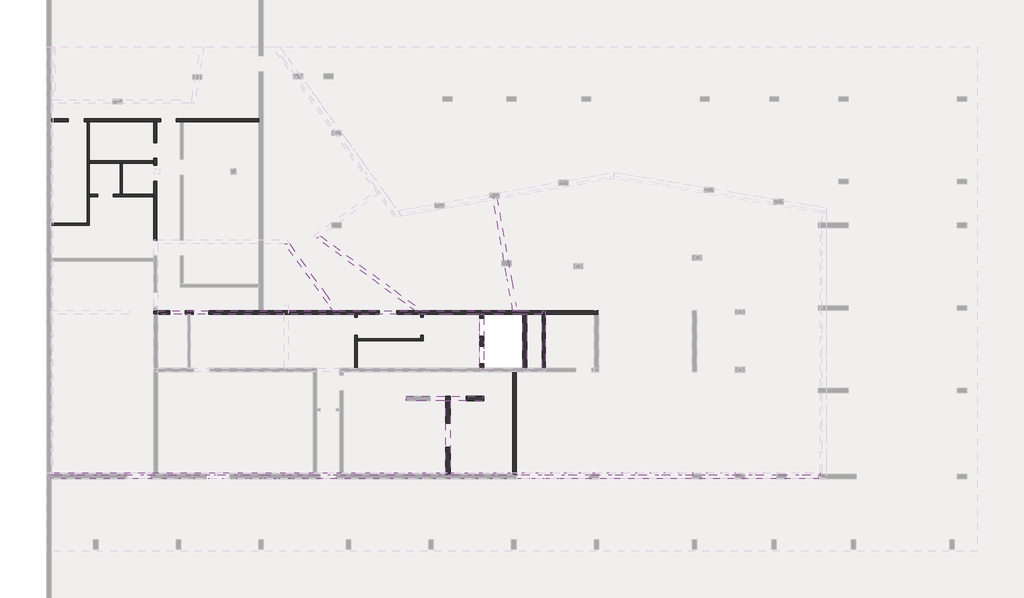
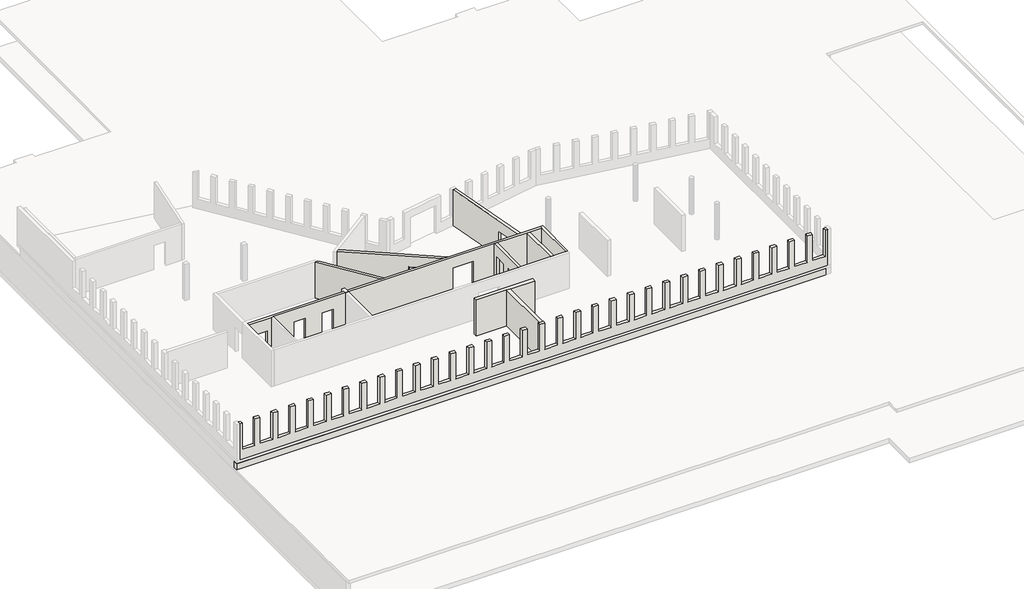
# One storey, part 2 of 4: 29 walls.
"""IFC4 building model written with IfcOpenShell, lengths in millimetres."""

from ifc_helpers import new_model, si_unit, frame, origin, place, context, project, spatial, polyline, outline, extrude, faceted_brep, element, save

model = new_model("IFC4")

# Units and contexts
model_context = context("Model", 3, world=origin())
ifc_project = project(units=[si_unit("LENGTHUNIT", "METRE", prefix="MILLI")], contexts=[model_context])

# Site, building, storey
site = spatial("IfcSite", under=ifc_project)
building = spatial("IfcBuilding", under=site)
storey = spatial("IfcBuildingStorey", under=building, Name="01_UG_OKFB_-4,20", Elevation=-4200.0)

# Walls
placement = place(None, origin())
element("IfcWall", 1, ObjectType="5dki Lochfassade 26cm C30/37", at=placement, inside=storey, context=model_context, shape_type="Brep", body=[
    faceted_brep([(49396.9999991, 130.0010483, 710.0), (49396.9999991, 130.0010483, 3060.0), (49603.9991101, 130.0010486, 3060.0), (49603.9991101, 130.0010486, -150.0), (25766.9999915, 130.0010117, -150.0), (25466.9999915, 130.0010113, -150.0), (130.0010047, 130.000972, -150.0), (130.0010047, 130.000972, 3060.0), (317.0000012, 130.0009723, 3060.0), (316.999997, 130.0009723, 710.0), (1397.0000012, 130.000974, 710.0), (1397.0000069, 130.000974, 3060.0), (1816.9999991, 130.0009747, 3060.0), (1817.0000028, 130.0009747, 710.0), (2896.9999991, 130.0009763, 710.0), (2897.0000017, 130.0009763, 3060.0), (3316.9999991, 130.000977, 3060.0), (3316.9999977, 130.000977, 710.0), (4396.9999991, 130.0009787, 710.0), (4396.9999966, 130.0009787, 3060.0), (4816.9999991, 130.0009793, 3060.0), (4816.9999991, 130.0009793, 710.0), (5896.9999991, 130.000981, 710.0), (5896.9999991, 130.000981, 3060.0), (6316.9999991, 130.0009816, 3060.0), (6316.9999991, 130.0009816, 710.0), (7396.9999991, 130.0009833, 710.0), (7396.9999991, 130.0009833, 3060.0), (7816.9999991, 130.0009839, 3060.0), (7816.9999991, 130.0009839, 710.0), (8896.9999991, 130.0009856, 710.0), (8896.9999991, 130.0009856, 3060.0), (9316.9999991, 130.0009863, 3060.0), (9316.9999991, 130.0009863, 710.0), (10396.9999991, 130.0009879, 710.0), (10396.9999991, 130.0009879, 3060.0), (10816.9999991, 130.0009886, 3060.0), (10816.9999991, 130.0009886, 710.0), (11896.9999991, 130.0009903, 710.0), (11896.9999991, 130.0009903, 3060.0), (12316.9999991, 130.0009909, 3060.0), (12316.9999991, 130.0009909, 710.0), (13396.9999991, 130.0009926, 710.0), (13396.9999991, 130.0009926, 3060.0), (13816.9999991, 130.0009932, 3060.0), (13816.9999991, 130.0009932, 710.0), (14896.9999991, 130.0009949, 710.0), (14896.9999991, 130.0009949, 3060.0), (15316.9999991, 130.0009956, 3060.0), (15316.9999991, 130.0009956, 710.0), (16396.9999991, 130.0009972, 710.0), (16396.9999991, 130.0009972, 3060.0), (16816.9999991, 130.0009979, 3060.0), (16816.9999991, 130.0009979, 710.0), (17896.9999991, 130.0009996, 710.0), (17896.9999991, 130.0009996, 3060.0), (18316.9999991, 130.0010002, 3060.0), (18316.9999991, 130.0010002, 710.0), (19396.9999991, 130.0010019, 710.0), (19396.9999991, 130.0010019, 3060.0), (19816.9999991, 130.0010025, 3060.0), (19816.9999991, 130.0010025, 710.0), (20896.9999991, 130.0010042, 710.0), (20896.9999991, 130.0010042, 3060.0), (21316.9999991, 130.0010048, 3060.0), (21316.9999991, 130.0010048, 710.0), (22396.9999991, 130.0010065, 710.0), (22396.9999991, 130.0010065, 3060.0), (22816.9999991, 130.0010072, 3060.0), (22816.9999991, 130.0010072, 710.0), (23896.9999991, 130.0010088, 710.0), (23896.9999991, 130.0010088, 3060.0), (24316.9999991, 130.0010095, 3060.0), (24316.9999991, 130.0010095, 710.0), (25396.9999991, 130.0010112, 710.0), (25396.9999991, 130.0010112, 3060.0), (25466.9999915, 130.0010113, 3060.0), (25766.9999915, 130.0010117, 3060.0), (25816.9999991, 130.0010118, 3060.0), (25816.9999991, 130.0010118, 710.0), (26896.9999991, 130.0010135, 710.0), (26896.9999991, 130.0010135, 3060.0), (27316.9999991, 130.0010141, 3060.0), (27316.9999991, 130.0010141, 710.0), (28396.9999991, 130.0010158, 710.0), (28396.9999991, 130.0010158, 3060.0), (28816.9999991, 130.0010165, 3060.0), (28816.9999991, 130.0010165, 710.0), (29896.9999991, 130.0010181, 710.0), (29896.9999991, 130.0010181, 3060.0), (30316.9999991, 130.0010188, 3060.0), (30316.9999991, 130.0010188, 710.0), (31396.9999991, 130.0010205, 710.0), (31396.9999991, 130.0010205, 3060.0), (31816.9999991, 130.0010211, 3060.0), (31816.9999991, 130.0010211, 710.0), (32896.9999991, 130.0010228, 710.0), (32896.9999991, 130.0010228, 3060.0), (33316.9999991, 130.0010234, 3060.0), (33316.9999991, 130.0010234, 710.0), (34396.9999991, 130.0010251, 710.0), (34396.9999991, 130.0010251, 3060.0), (34816.9999991, 130.0010258, 3060.0), (34816.9999991, 130.0010258, 710.0), (35896.9999991, 130.0010274, 710.0), (35896.9999991, 130.0010274, 3060.0), (36316.9999991, 130.0010281, 3060.0), (36316.9999991, 130.0010281, 710.0), (37396.9999991, 130.0010297, 710.0), (37396.9999991, 130.0010297, 3060.0), (37816.9999991, 130.0010304, 3060.0), (37816.9999991, 130.0010304, 710.0), (38896.9999991, 130.0010321, 710.0), (38896.9999991, 130.0010321, 3060.0), (39316.9999991, 130.0010327, 3060.0), (39316.9999991, 130.0010327, 710.0), (40396.9999991, 130.0010344, 710.0), (40396.9999991, 130.0010344, 3060.0), (40816.9999991, 130.001035, 3060.0), (40816.9999991, 130.001035, 710.0), (41896.9999991, 130.0010367, 710.0), (41896.9999991, 130.0010367, 3060.0), (42316.9999991, 130.0010374, 3060.0), (42316.9999991, 130.0010374, 710.0), (43396.9999991, 130.001039, 710.0), (43396.9999991, 130.001039, 3060.0), (43816.9999991, 130.0010397, 3060.0), (43816.9999991, 130.0010397, 710.0), (44896.9999991, 130.0010414, 710.0), (44896.9999991, 130.0010414, 3060.0), (45316.9999991, 130.001042, 3060.0), (45316.9999991, 130.001042, 710.0), (46396.9999991, 130.0010437, 710.0), (46396.9999991, 130.0010437, 3060.0), (46816.9999991, 130.0010443, 3060.0), (46816.9999991, 130.0010443, 710.0), (47896.9999991, 130.001046, 710.0), (47896.9999991, 130.001046, 3060.0), (48316.9999991, 130.0010467, 3060.0), (48316.9999991, 130.0010467, 710.0), (49603.9991105, -129.9989514, 3060.0), (49396.9999995, -129.9989517, 3060.0), (49396.9999995, -129.9989517, 710.0), (48316.9999995, -129.9989533, 710.0), (48316.9999995, -129.9989533, 3060.0), (47896.9999995, -129.998954, 3060.0), (47896.9999995, -129.998954, 710.0), (46816.9999995, -129.9989557, 710.0), (46816.9999995, -129.9989557, 3060.0), (46396.9999995, -129.9989563, 3060.0), (46396.9999995, -129.9989563, 710.0), (45316.9999995, -129.998958, 710.0), (45316.9999995, -129.998958, 3060.0), (44896.9999995, -129.9989586, 3060.0), (44896.9999995, -129.9989586, 710.0), (43816.9999995, -129.9989603, 710.0), (43816.9999995, -129.9989603, 3060.0), (43396.9999995, -129.998961, 3060.0), (43396.9999995, -129.998961, 710.0), (42316.9999995, -129.9989626, 710.0), (42316.9999995, -129.9989626, 3060.0), (41896.9999995, -129.9989633, 3060.0), (41896.9999995, -129.9989633, 710.0), (40816.9999995, -129.998965, 710.0), (40816.9999995, -129.998965, 3060.0), (40396.9999995, -129.9989656, 3060.0), (40396.9999995, -129.9989656, 710.0), (39316.9999995, -129.9989673, 710.0), (39316.9999995, -129.9989673, 3060.0), (38896.9999995, -129.9989679, 3060.0), (38896.9999995, -129.9989679, 710.0), (37816.9999995, -129.9989696, 710.0), (37816.9999995, -129.9989696, 3060.0), (37396.9999995, -129.9989703, 3060.0), (37396.9999995, -129.9989703, 710.0), (36316.9999995, -129.9989719, 710.0), (36316.9999995, -129.9989719, 3060.0), (35896.9999995, -129.9989726, 3060.0), (35896.9999995, -129.9989726, 710.0), (34816.9999995, -129.9989742, 710.0), (34816.9999995, -129.9989742, 3060.0), (34396.9999995, -129.9989749, 3060.0), (34396.9999995, -129.9989749, 710.0), (33316.9999995, -129.9989766, 710.0), (33316.9999995, -129.9989766, 3060.0), (32896.9999995, -129.9989772, 3060.0), (32896.9999995, -129.9989772, 710.0), (31816.9999995, -129.9989789, 710.0), (31816.9999995, -129.9989789, 3060.0), (31396.9999995, -129.9989795, 3060.0), (31396.9999995, -129.9989795, 710.0), (30316.9999995, -129.9989812, 710.0), (30316.9999995, -129.9989812, 3060.0), (29896.9999995, -129.9989819, 3060.0), (29896.9999995, -129.9989819, 710.0), (28816.9999995, -129.9989835, 710.0), (28816.9999995, -129.9989835, 3060.0), (28396.9999995, -129.9989842, 3060.0), (28396.9999995, -129.9989842, 710.0), (27316.9999995, -129.9989859, 710.0), (27316.9999995, -129.9989859, 3060.0), (26896.9999995, -129.9989865, 3060.0), (26896.9999995, -129.9989865, 710.0), (25816.9999995, -129.9989882, 710.0), (25816.9999995, -129.9989882, 3060.0), (25396.9999995, -129.9989888, 3060.0), (25396.9999995, -129.9989888, 710.0), (24316.9999995, -129.9989905, 710.0), (24316.9999995, -129.9989905, 3060.0), (23896.9999995, -129.9989912, 3060.0), (23896.9999995, -129.9989912, 710.0), (22816.9999995, -129.9989928, 710.0), (22816.9999995, -129.9989928, 3060.0), (22396.9999995, -129.9989935, 3060.0), (22396.9999995, -129.9989935, 710.0), (21316.9999995, -129.9989952, 710.0), (21316.9999995, -129.9989952, 3060.0), (20896.9999995, -129.9989958, 3060.0), (20896.9999995, -129.9989958, 710.0), (19816.9999995, -129.9989975, 710.0), (19816.9999995, -129.9989975, 3060.0), (19396.9999995, -129.9989981, 3060.0), (19396.9999995, -129.9989981, 710.0), (18316.9999995, -129.9989998, 710.0), (18316.9999995, -129.9989998, 3060.0), (17896.9999995, -129.9990004, 3060.0), (17896.9999995, -129.9990004, 710.0), (16816.9999995, -129.9990021, 710.0), (16816.9999995, -129.9990021, 3060.0), (16396.9999995, -129.9990028, 3060.0), (16396.9999995, -129.9990028, 710.0), (15316.9999995, -129.9990044, 710.0), (15316.9999995, -129.9990044, 3060.0), (14896.9999995, -129.9990051, 3060.0), (14896.9999995, -129.9990051, 710.0), (13816.9999995, -129.9990068, 710.0), (13816.9999995, -129.9990068, 3060.0), (13396.9999995, -129.9990074, 3060.0), (13396.9999995, -129.9990074, 710.0), (12316.9999995, -129.9990091, 710.0), (12316.9999995, -129.9990091, 3060.0), (11896.9999995, -129.9990097, 3060.0), (11896.9999995, -129.9990097, 710.0), (10816.9999995, -129.9990114, 710.0), (10816.9999995, -129.9990114, 3060.0), (10396.9999995, -129.9990121, 3060.0), (10396.9999995, -129.9990121, 710.0), (9316.9999995, -129.9990137, 710.0), (9316.9999995, -129.9990137, 3060.0), (8896.9999995, -129.9990144, 3060.0), (8896.9999995, -129.9990144, 710.0), (7816.9999995, -129.9990161, 710.0), (7816.9999995, -129.9990161, 3060.0), (7396.9999995, -129.9990167, 3060.0), (7396.9999995, -129.9990167, 710.0), (6316.9999995, -129.9990184, 710.0), (6316.9999995, -129.9990184, 3060.0), (5896.9999995, -129.999019, 3060.0), (5896.9999995, -129.999019, 710.0), (4816.9999995, -129.9990207, 710.0), (4816.9999995, -129.9990207, 3060.0), (4396.9999995, -129.9990213, 3060.0), (4396.9999966, -129.9990213, 710.0), (3316.9999995, -129.999023, 710.0), (3316.9999977, -129.999023, 3060.0), (2896.9999995, -129.9990237, 3060.0), (2897.0000017, -129.9990237, 710.0), (1816.9999995, -129.9990253, 710.0), (1817.0000028, -129.9990253, 3060.0), (1397.0000016, -129.999026, 3060.0), (1397.0000069, -129.999026, 710.0), (317.0000016, -129.9990277, 710.0), (316.999997, -129.9990277, 3060.0), (130.0010047, -129.999028, 3060.0), (130.0010047, -129.999028, -150.0), (49603.9991105, -129.9989514, -150.0)], [[[0, 1, 2, 3, 4, 5, 6, 7, 8, 9, 10, 11, 12, 13, 14, 15, 16, 17, 18, 19, 20, 21, 22, 23, 24, 25, 26, 27, 28, 29, 30, 31, 32, 33, 34, 35, 36, 37, 38, 39, 40, 41, 42, 43, 44, 45, 46, 47, 48, 49, 50, 51, 52, 53, 54, 55, 56, 57, 58, 59, 60, 61, 62, 63, 64, 65, 66, 67, 68, 69, 70, 71, 72, 73, 74, 75, 76, 77, 78, 79, 80, 81, 82, 83, 84, 85, 86, 87, 88, 89, 90, 91, 92, 93, 94, 95, 96, 97, 98, 99, 100, 101, 102, 103, 104, 105, 106, 107, 108, 109, 110, 111, 112, 113, 114, 115, 116, 117, 118, 119, 120, 121, 122, 123, 124, 125, 126, 127, 128, 129, 130, 131, 132, 133, 134, 135, 136, 137, 138, 139]], [[140, 141, 142, 143, 144, 145, 146, 147, 148, 149, 150, 151, 152, 153, 154, 155, 156, 157, 158, 159, 160, 161, 162, 163, 164, 165, 166, 167, 168, 169, 170, 171, 172, 173, 174, 175, 176, 177, 178, 179, 180, 181, 182, 183, 184, 185, 186, 187, 188, 189, 190, 191, 192, 193, 194, 195, 196, 197, 198, 199, 200, 201, 202, 203, 204, 205, 206, 207, 208, 209, 210, 211, 212, 213, 214, 215, 216, 217, 218, 219, 220, 221, 222, 223, 224, 225, 226, 227, 228, 229, 230, 231, 232, 233, 234, 235, 236, 237, 238, 239, 240, 241, 242, 243, 244, 245, 246, 247, 248, 249, 250, 251, 252, 253, 254, 255, 256, 257, 258, 259, 260, 261, 262, 263, 264, 265, 266, 267, 268, 269, 270, 271, 272, 273, 274, 275]], [[6, 5, 4, 3, 275, 274]], [[7, 273, 272, 8]], [[15, 265, 264, 16]], [[268, 12, 11, 269]], [[261, 260, 20, 19]], [[257, 256, 24, 23]], [[253, 252, 28, 27]], [[249, 248, 32, 31]], [[245, 244, 36, 35]], [[241, 240, 40, 39]], [[237, 236, 44, 43]], [[233, 232, 48, 47]], [[229, 228, 52, 51]], [[225, 224, 56, 55]], [[221, 220, 60, 59]], [[217, 216, 64, 63]], [[213, 212, 68, 67]], [[209, 208, 72, 71]], [[205, 204, 78, 77, 76, 75]], [[201, 200, 82, 81]], [[197, 196, 86, 85]], [[193, 192, 90, 89]], [[189, 188, 94, 93]], [[185, 184, 98, 97]], [[181, 180, 102, 101]], [[177, 176, 106, 105]], [[173, 172, 110, 109]], [[169, 168, 114, 113]], [[165, 164, 118, 117]], [[161, 160, 122, 121]], [[157, 156, 126, 125]], [[153, 152, 130, 129]], [[149, 148, 134, 133]], [[138, 137, 145, 144]], [[2, 1, 141, 140]], [[7, 6, 274, 273]], [[3, 2, 140, 275]], [[10, 270, 269, 11]], [[271, 9, 8, 272]], [[270, 10, 9, 271]], [[14, 266, 265, 15]], [[267, 13, 12, 268]], [[266, 14, 13, 267]], [[18, 262, 261, 19]], [[263, 17, 16, 264]], [[262, 18, 17, 263]], [[23, 22, 258, 257]], [[21, 20, 260, 259]], [[22, 21, 259, 258]], [[27, 26, 254, 253]], [[25, 24, 256, 255]], [[26, 25, 255, 254]], [[31, 30, 250, 249]], [[29, 28, 252, 251]], [[30, 29, 251, 250]], [[35, 34, 246, 245]], [[33, 32, 248, 247]], [[34, 33, 247, 246]], [[39, 38, 242, 241]], [[37, 36, 244, 243]], [[38, 37, 243, 242]], [[43, 42, 238, 237]], [[41, 40, 240, 239]], [[42, 41, 239, 238]], [[47, 46, 234, 233]], [[45, 44, 236, 235]], [[46, 45, 235, 234]], [[51, 50, 230, 229]], [[49, 48, 232, 231]], [[50, 49, 231, 230]], [[55, 54, 226, 225]], [[53, 52, 228, 227]], [[54, 53, 227, 226]], [[59, 58, 222, 221]], [[57, 56, 224, 223]], [[58, 57, 223, 222]], [[63, 62, 218, 217]], [[61, 60, 220, 219]], [[62, 61, 219, 218]], [[67, 66, 214, 213]], [[65, 64, 216, 215]], [[66, 65, 215, 214]], [[71, 70, 210, 209]], [[69, 68, 212, 211]], [[70, 69, 211, 210]], [[75, 74, 206, 205]], [[73, 72, 208, 207]], [[74, 73, 207, 206]], [[81, 80, 202, 201]], [[79, 78, 204, 203]], [[80, 79, 203, 202]], [[85, 84, 198, 197]], [[83, 82, 200, 199]], [[84, 83, 199, 198]], [[89, 88, 194, 193]], [[87, 86, 196, 195]], [[88, 87, 195, 194]], [[93, 92, 190, 189]], [[91, 90, 192, 191]], [[92, 91, 191, 190]], [[97, 96, 186, 185]], [[95, 94, 188, 187]], [[96, 95, 187, 186]], [[101, 100, 182, 181]], [[99, 98, 184, 183]], [[100, 99, 183, 182]], [[105, 104, 178, 177]], [[103, 102, 180, 179]], [[104, 103, 179, 178]], [[109, 108, 174, 173]], [[107, 106, 176, 175]], [[108, 107, 175, 174]], [[113, 112, 170, 169]], [[111, 110, 172, 171]], [[112, 111, 171, 170]], [[117, 116, 166, 165]], [[115, 114, 168, 167]], [[116, 115, 167, 166]], [[121, 120, 162, 161]], [[119, 118, 164, 163]], [[120, 119, 163, 162]], [[125, 124, 158, 157]], [[123, 122, 160, 159]], [[124, 123, 159, 158]], [[129, 128, 154, 153]], [[127, 126, 156, 155]], [[128, 127, 155, 154]], [[133, 132, 150, 149]], [[131, 130, 152, 151]], [[132, 131, 151, 150]], [[137, 136, 146, 145]], [[135, 134, 148, 147]], [[136, 135, 147, 146]], [[144, 143, 139, 138]], [[142, 141, 1, 0]], [[143, 142, 0, 139]]]),
])
element("IfcWall", 2, ObjectType="5dki STB-Wand Kern 25cm C30/37", at=placement, inside=storey, context=model_context, shape_type="Brep", body=[
    faceted_brep([(18223.2182524, 10662.0127257, 3060.0), (15141.8279932, 14942.0124447, 3060.0), (15141.8279932, 14942.0124447, -150.0), (17305.3310134, 11936.9428041, -150.0), (17305.3310134, 11936.9428041, 1985.0), (17895.4523577, 11117.2740911, 1985.0), (17895.4523577, 11117.2740911, -150.0), (18223.2182524, 10662.0127257, -150.0), (15449.8792779, 14942.0124447, 3060.0), (18531.2695366, 10662.0127262, 3060.0), (18531.2695366, 10662.0127262, -150.0), (18098.340653, 11263.3437308, -150.0), (18098.340653, 11263.3437308, 1985.0), (17508.2193087, 12083.0124438, 1985.0), (17508.2193087, 12083.0124438, -150.0), (15449.8792779, 14942.0124447, -150.0)], [[[0, 1, 2, 3, 4, 5, 6, 7]], [[8, 9, 10, 11, 12, 13, 14, 15]], [[2, 15, 14, 3]], [[10, 7, 6, 11]], [[1, 0, 9, 8]], [[2, 1, 8, 15]], [[0, 7, 10, 9]], [[13, 4, 3, 14]], [[4, 13, 12, 5]], [[5, 12, 11, 6]]]),
])
element("IfcWall", 3, ObjectType="5dki STB-Wand Kern 25cm C30/37", at=placement, inside=storey, context=model_context, shape_type="SweptSolid", body=[
    extrude(outline(polyline([(30641.9999891, 10442.0127483), (30641.9999891, 6960.0000501), (30391.9999891, 6960.0000498), (30391.9999891, 10442.0127479), (30641.9999891, 10442.0127483)])), frame((0.0, 0.0, -150.0), z_axis=(0.0, 0.0, 1.0), x_axis=(1.0, 0.0, 0.0)), (0.0, 0.0, 1.0), 3210.0),
])
element("IfcWall", 4, ObjectType="5dki STB-Wand Kern 25cm C30/37", at=placement, inside=storey, context=model_context, shape_type="SweptSolid", body=[
    extrude(outline(polyline([(3482.0126944, -3210.0), (-2.1e-06, -3210.0), (-2.1e-06, 0.0), (279.9681323, 0.0), (279.9681323, -2260.0), (1414.9681323, -2260.0), (1414.9681323, 0.0), (2067.1995869, 0.0), (2067.1995869, -2260.0), (3202.1995869, -2260.0), (3202.1995869, 0.0), (3482.0126944, 0.0), (3482.0126944, -3210.0)])), frame((27641.9999829, 10442.0127408, -150.0), z_axis=(1.0, 1.6300916066412081e-09, 0.0), x_axis=(1.6300916066412081e-09, -1.0, 0.0)), (0.0, 0.0, 1.0), 250.0),
])
element("IfcWall", 5, ObjectType="5dki STB-Wand Kern 20cm C35/45", at=placement, inside=storey, context=model_context, shape_type="Brep", body=[
    faceted_brep([(31641.9999912, 10662.0127502, -150.0), (31641.9999881, 10442.0127502, -150.0), (31641.9999382, 6960.0000514, -150.0), (31641.9999382, 6960.0000514, 3060.0), (31641.9999881, 10442.0127502, 3060.0), (31641.9999912, 10662.0127502, 3060.0), (31841.9999912, 10662.0127505, -150.0), (31841.9999912, 10662.0127505, 3060.0), (31841.9999382, 6960.0000516, 3060.0), (31841.9999382, 6960.0000516, -150.0)], [[[0, 1, 2, 3, 4, 5]], [[6, 7, 8, 9]], [[2, 1, 0, 6, 9]], [[5, 4, 3, 8, 7]], [[0, 5, 7, 6]], [[3, 2, 9, 8]]]),
])
element("IfcWall", 6, ObjectType="5dki STB-Wand Kern 22cm C30/37", at=placement, inside=storey, context=model_context, shape_type="Brep", body=[
    faceted_brep([(6989.9995723, 10662.0127052, 3060.0), (18223.2182524, 10662.0127257, 3060.0), (18531.2695366, 10662.0127262, 3060.0), (23491.8764947, 10662.0127353, 3060.0), (23912.428752, 10662.0127361, 3060.0), (29768.165987, 10662.0127467, 3060.0), (30022.0739196, 10662.0127472, 3060.0), (31641.9999912, 10662.0127502, 3060.0), (31641.9999912, 10662.0127502, -150.0), (30022.0739196, 10662.0127472, -150.0), (29768.165987, 10662.0127467, -150.0), (25926.999945, 10662.0127397, -150.0), (25927.0000254, 10662.0127397, 2110.0), (24166.999945, 10662.0127365, 2110.0), (24166.9998144, 10662.0127365, -150.0), (23912.428752, 10662.0127361, -150.0), (23491.8764947, 10662.0127353, -150.0), (18531.2695366, 10662.0127262, -150.0), (18223.2182524, 10662.0127257, -150.0), (14152.0004935, 10662.0127182, -150.0), (14152.0007698, 10662.0127182, 1985.0), (13142.0004935, 10662.0127164, 1985.0), (13142.0009721, 10662.0127164, -150.0), (11796.9999806, 10662.0127139, -150.0), (11796.9997327, 10662.0127139, 1985.0), (10786.9999806, 10662.0127121, 1985.0), (10786.999935, 10662.0127121, -150.0), (8540.0010342, 10662.012708, -150.0), (8540.000485, 10662.012708, 1985.0), (7530.0010342, 10662.0127061, 1985.0), (7530.0006873, 10662.0127061, -150.0), (6989.9995723, 10662.0127052, -150.0), (31641.9999881, 10442.0127502, 3060.0), (30641.9999891, 10442.0127483, 3060.0), (30391.9999891, 10442.0127479, 3060.0), (27891.9999829, 10442.0127433, 3060.0), (27641.9999829, 10442.0127429, 3060.0), (9066.9999886, 10442.0127089, 3060.0), (8916.9999886, 10442.0127087, 3060.0), (6989.9995723, 10442.0127052, 3060.0), (6989.9995723, 10442.0127052, -150.0), (7530.0010346, 10442.0127061, -150.0), (7530.0006873, 10442.0127061, 1985.0), (8540.0010346, 10442.012708, 1985.0), (8540.000485, 10442.012708, -150.0), (8916.9999886, 10442.0127087, -150.0), (9066.9999886, 10442.0127089, -150.0), (10786.999981, 10442.0127121, -150.0), (10786.999935, 10442.0127121, 1985.0), (11796.999981, 10442.0127139, 1985.0), (11796.9997327, 10442.0127139, -150.0), (13142.0004939, 10442.0127164, -150.0), (13142.0009721, 10442.0127164, 1985.0), (14152.0004939, 10442.0127182, 1985.0), (14152.0007698, 10442.0127182, -150.0), (24166.9999454, 10442.0127365, -150.0), (24166.9998144, 10442.0127365, 2110.0), (25926.9999454, 10442.0127397, 2110.0), (25927.0000254, 10442.0127397, -150.0), (27641.9999829, 10442.0127429, -150.0), (27891.9999829, 10442.0127433, -150.0), (30391.9999891, 10442.0127479, -150.0), (30641.9999891, 10442.0127483, -150.0), (31641.9999881, 10442.0127502, -150.0)], [[[0, 1, 2, 3, 4, 5, 6, 7, 8, 9, 10, 11, 12, 13, 14, 15, 16, 17, 18, 19, 20, 21, 22, 23, 24, 25, 26, 27, 28, 29, 30, 31]], [[32, 33, 34, 35, 36, 37, 38, 39, 40, 41, 42, 43, 44, 45, 46, 47, 48, 49, 50, 51, 52, 53, 54, 55, 56, 57, 58, 59, 60, 61, 62, 63]], [[40, 31, 30, 41]], [[8, 63, 62, 61, 60, 59, 58, 11, 10, 9]], [[14, 55, 54, 19, 18, 17, 16, 15]], [[26, 47, 46, 45, 44, 27]], [[50, 23, 22, 51]], [[7, 6, 5, 4, 3, 2, 1, 0, 39, 38, 37, 36, 35, 34, 33, 32]], [[0, 31, 40, 39]], [[8, 7, 32, 63]], [[57, 12, 11, 58]], [[12, 57, 56, 13]], [[13, 56, 55, 14]], [[25, 48, 47, 26]], [[48, 25, 24, 49]], [[49, 24, 23, 50]], [[21, 52, 51, 22]], [[52, 21, 20, 53]], [[53, 20, 19, 54]], [[29, 42, 41, 30]], [[42, 29, 28, 43]], [[43, 28, 27, 44]]]),
])
element("IfcWall", 7, ObjectType="5dki STB-Wand Kern 22cm C30/37", at=placement, inside=storey, context=model_context, shape_type="Brep", body=[
    faceted_brep([(35269.9993003, 10442.0122959, -400.0), (6740.0003427, 10442.0129553, -400.0), (6740.0003427, 10442.0129553, -1200.0), (6740.0003427, 10442.0129553, -4200.0), (6990.0003427, 10442.0129495, -4200.0), (7756.9991752, 10442.0129318, -4200.0), (7756.999089, 10442.0129318, -2065.0), (8766.9991752, 10442.0129085, -2065.0), (8766.9991332, 10442.0129085, -4200.0), (8916.9991145, 10442.012905, -4200.0), (9066.9991145, 10442.0129015, -4200.0), (9266.9991145, 10442.0128969, -4200.0), (9266.9990345, 10442.0128969, -2065.0), (10276.9991145, 10442.0128736, -2065.0), (10276.9990788, 10442.0128736, -4200.0), (19626.9996762, 10442.0126575, -4200.0), (19776.9996762, 10442.012654, -4200.0), (21192.0596983, 10442.0126213, -4200.0), (21192.0596059, 10442.0126213, -1940.0), (22327.0596983, 10442.0125951, -1940.0), (22327.0596723, 10442.0125951, -4200.0), (23856.9975771, 10442.0125597, -4200.0), (24006.9975771, 10442.0125562, -4200.0), (27642.000202, 10442.0124722, -4200.0), (27892.000202, 10442.0124665, -4200.0), (30391.9991141, 10442.0124087, -4200.0), (30641.9991141, 10442.0124029, -4200.0), (31641.9991989, 10442.0123798, -4200.0), (31841.9991989, 10442.0123752, -4200.0), (34969.9993003, 10442.0123029, -4200.0), (35269.9993003, 10442.0122959, -4200.0), (35269.9993003, 10442.0122959, -1200.0), (6740.000326, 10662.0129553, -400.0), (35269.9992997, 10662.0122959, -400.0), (35269.9992997, 10662.0122959, -4200.0), (22327.0597034, 10662.0125951, -4200.0), (22327.0596723, 10662.0125951, -1940.0), (21192.0597034, 10662.0126213, -1940.0), (21192.0596059, 10662.0126213, -4200.0), (13769.9992195, 10662.0127928, -4200.0), (13469.9992195, 10662.0127998, -4200.0), (10276.9991196, 10662.0128736, -4200.0), (10276.9990788, 10662.0128736, -2065.0), (9266.9991196, 10662.0128969, -2065.0), (9266.9990345, 10662.0128969, -4200.0), (8766.9991803, 10662.0129085, -4200.0), (8766.9991332, 10662.0129085, -2065.0), (7756.9991803, 10662.0129318, -2065.0), (7756.999089, 10662.0129318, -4200.0), (6939.9999661, 10662.0129507, -4200.0), (6740.000326, 10662.0129553, -4200.0), (6740.000326, 10662.0129553, -1200.0)], [[[0, 1, 2, 3, 4, 5, 6, 7, 8, 9, 10, 11, 12, 13, 14, 15, 16, 17, 18, 19, 20, 21, 22, 23, 24, 25, 26, 27, 28, 29, 30, 31]], [[32, 33, 34, 35, 36, 37, 38, 39, 40, 41, 42, 43, 44, 45, 46, 47, 48, 49, 50, 51]], [[34, 30, 29, 28, 27, 26, 25, 24, 23, 22, 21, 20, 35]], [[3, 50, 49, 48, 5, 4]], [[38, 17, 16, 15, 14, 41, 40, 39]], [[44, 11, 10, 9, 8, 45]], [[1, 0, 33, 32]], [[0, 31, 30, 34, 33]], [[3, 2, 1, 32, 51, 50]], [[37, 18, 17, 38]], [[18, 37, 36, 19]], [[19, 36, 35, 20]], [[13, 42, 41, 14]], [[42, 13, 12, 43]], [[43, 12, 11, 44]], [[7, 46, 45, 8]], [[46, 7, 6, 47]], [[47, 6, 5, 48]]]),
])
element("IfcWall", 8, ObjectType="5dki STB-Wand Kern 20cm C35/45", at=placement, inside=storey, context=model_context, shape_type="SweptSolid", body=[
    extrude(outline(polyline([(31641.9991143, 6960.0014903), (31641.9991989, 10442.0123798), (31841.9991989, 10442.0123752), (31841.9991143, 6960.0015008), (31641.9991143, 6960.0014903)])), frame((0.0, 0.0, -4200.0), z_axis=(0.0, 0.0, 1.0), x_axis=(1.0, 0.0, 0.0)), (0.0, 0.0, 1.0), 3000.0),
])
element("IfcWall", 9, ObjectType="5dki STB-Wand Kern 25cm C30/37", at=placement, inside=storey, context=model_context, shape_type="SweptSolid", body=[
    extrude(outline(polyline([(30391.9991141, 6960.0014246), (30391.9991141, 10442.0124087), (30641.9991141, 10442.0124029), (30641.9991141, 6960.0014377), (30391.9991141, 6960.0014246)])), frame((0.0, 0.0, -4200.0), z_axis=(0.0, 0.0, 1.0), x_axis=(1.0, 0.0, 0.0)), (0.0, 0.0, 1.0), 3000.0),
])
element("IfcWall", 10, ObjectType="5dki STB-Wand Kern 25cm C30/37", at=placement, inside=storey, context=model_context, shape_type="Brep", body=[
    faceted_brep([(27642.0002944, 6960.0012801, -1200.0), (27642.000202, 10442.0124722, -1200.0), (27642.000202, 10442.0124722, -4200.0), (27642.0002094, 10162.0446386, -4200.0), (27642.0002094, 10162.0446386, -1940.0), (27642.0002395, 9027.0446386, -1940.0), (27642.0002395, 9027.0446386, -4200.0), (27642.0002568, 8374.9562225, -4200.0), (27642.0002568, 8374.9562225, -1940.0), (27642.000287, 7239.9562225, -1940.0), (27642.000287, 7239.9562225, -4200.0), (27642.0002944, 6960.0012801, -4200.0), (27892.000202, 10442.0124665, -1200.0), (27892.0002944, 6960.0012933, -1200.0), (27892.0002944, 6960.0012933, -4200.0), (27892.000287, 7239.9562292, -4200.0), (27892.000287, 7239.9562292, -1940.0), (27892.0002568, 8374.9562292, -1940.0), (27892.0002568, 8374.9562292, -4200.0), (27892.0002395, 9027.0446452, -4200.0), (27892.0002395, 9027.0446452, -1940.0), (27892.0002094, 10162.0446452, -1940.0), (27892.0002094, 10162.0446452, -4200.0), (27892.000202, 10442.0124665, -4200.0)], [[[0, 1, 2, 3, 4, 5, 6, 7, 8, 9, 10, 11]], [[12, 13, 14, 15, 16, 17, 18, 19, 20, 21, 22, 23]], [[2, 23, 22, 3]], [[14, 11, 10, 15]], [[6, 19, 18, 7]], [[1, 0, 13, 12]], [[2, 1, 12, 23]], [[0, 11, 14, 13]], [[21, 4, 3, 22]], [[4, 21, 20, 5]], [[5, 20, 19, 6]], [[9, 16, 15, 10]], [[16, 9, 8, 17]], [[17, 8, 7, 18]]]),
])
element("IfcWall", 11, ObjectType="5dki Überzug 40cm C30/37", at=placement, inside=storey, context=model_context, shape_type="Brep", body=[
    faceted_brep([(49463.9991099, 270.0010491, -950.0), (-130.0001888, 270.0010491, -950.0), (-130.0001888, 270.0010491, -400.0), (269.9998112, 270.0010491, -400.0), (49463.9991099, 270.0010491, -400.0), (49463.9991105, -129.9989509, -950.0), (49463.9991105, -129.9989509, -400.0), (-130.0001888, -129.9989509, -400.0), (-130.0001888, -129.9989509, -950.0)], [[[0, 1, 2, 3, 4]], [[5, 6, 7, 8]], [[1, 0, 5, 8]], [[4, 3, 2, 7, 6]], [[0, 4, 6, 5]], [[2, 1, 8, 7]]]),
])
element("IfcWall", 12, ObjectType="5dki STB-Wand 15cm C20/25", at=placement, inside=storey, context=model_context, shape_type="Brep", body=[
    faceted_brep([(171.303059, 16118.6537915, -4200.0), (2620.0006409, 16118.6537287, -4200.0), (2620.0006409, 16118.6537287, -1200.0), (171.303059, 16118.6537915, -1200.0), (171.3030629, 16268.6537915, -4200.0), (171.3030629, 16268.6537915, -1200.0), (2470.0006409, 16268.6537326, -1200.0), (2620.0006409, 16268.6537287, -1200.0), (2620.0006409, 16268.6537287, -4200.0), (2470.0006409, 16268.6537326, -4200.0)], [[[0, 1, 2, 3]], [[4, 5, 6, 7, 8, 9]], [[1, 0, 4, 9, 8]], [[3, 2, 7, 6, 5]], [[0, 3, 5, 4]], [[2, 1, 8, 7]]]),
])
element("IfcWall", 13, ObjectType="5dki STB-Wand 15cm C20/25", at=placement, inside=storey, context=model_context, shape_type="Brep", body=[
    faceted_brep([(2620.0006409, 16268.6537287, -4200.0), (2620.0006409, 17969.9813796, -4200.0), (2620.0006409, 18119.9813796, -4200.0), (2620.0006409, 20119.9813888, -4200.0), (2620.0006409, 20269.9813888, -4200.0), (2620.0006409, 22768.6537287, -4200.0), (2620.0006409, 22768.6537287, -1200.0), (2620.0006409, 20269.9813888, -1200.0), (2620.0006409, 20119.9813888, -1200.0), (2620.0006409, 18119.9813796, -1200.0), (2620.0006409, 17969.9813796, -1200.0), (2620.0006409, 16268.6537287, -1200.0), (2470.0006409, 16268.6537326, -4200.0), (2470.0006409, 16268.6537326, -1200.0), (2470.0006409, 22768.6537287, -1200.0), (2470.0006409, 22768.6537287, -4200.0)], [[[0, 1, 2, 3, 4, 5, 6, 7, 8, 9, 10, 11]], [[12, 13, 14, 15]], [[5, 4, 3, 2, 1, 0, 12, 15]], [[6, 5, 15, 14]], [[11, 10, 9, 8, 7, 6, 14, 13]], [[0, 11, 13, 12]]]),
])
element("IfcWall", 14, ObjectType="5dki STB-Wand 15cm C20/25", at=placement, inside=storey, context=model_context, shape_type="Brep", body=[
    faceted_brep([(2620.0006409, 18119.9813796, -1200.0), (4580.0004286, 18119.9813362, -1200.0), (4730.0004286, 18119.9813329, -1200.0), (6740.0001703, 18119.9812884, -1200.0), (6740.0001703, 18119.9812884, -4200.0), (4730.0004286, 18119.9813329, -4200.0), (4580.0004286, 18119.9813362, -4200.0), (4147.4994555, 18119.9813458, -4200.0), (4147.4994814, 18119.9813458, -2065.0), (3137.4994555, 18119.9813681, -2065.0), (3137.4994853, 18119.9813681, -4200.0), (2620.0006409, 18119.9813796, -4200.0), (6740.0001663, 17969.9812884, -1200.0), (2620.0006409, 17969.9813796, -1200.0), (2620.0006409, 17969.9813796, -4200.0), (3137.4994522, 17969.9813681, -4200.0), (3137.4994853, 17969.9813681, -2065.0), (4147.4994522, 17969.9813458, -2065.0), (4147.4994814, 17969.9813458, -4200.0), (6740.0001663, 17969.9812884, -4200.0)], [[[0, 1, 2, 3, 4, 5, 6, 7, 8, 9, 10, 11]], [[12, 13, 14, 15, 16, 17, 18, 19]], [[14, 11, 10, 15]], [[4, 19, 18, 7, 6, 5]], [[3, 2, 1, 0, 13, 12]], [[0, 11, 14, 13]], [[4, 3, 12, 19]], [[9, 16, 15, 10]], [[16, 9, 8, 17]], [[17, 8, 7, 18]]]),
])
element("IfcWall", 15, ObjectType="5dki STB-Wand 15cm C20/25", at=placement, inside=storey, context=model_context, shape_type="SweptSolid", body=[
    extrude(outline(polyline([(4730.0004835, 20119.9813364), (4730.0004286, 18119.9813329), (4580.0004286, 18119.9813362), (4580.0004835, 20119.9813402), (4730.0004835, 20119.9813364)])), frame((0.0, 0.0, -4200.0), z_axis=(0.0, 0.0, 1.0), x_axis=(1.0, 0.0, 0.0)), (0.0, 0.0, 1.0), 3000.0),
])
element("IfcWall", 16, ObjectType="5dki STB-Wand 15cm C20/25", at=placement, inside=storey, context=model_context, shape_type="Brep", body=[
    faceted_brep([(2620.0006409, 20119.9813888, -4200.0), (4580.0004835, 20119.9813402, -4200.0), (4730.0004835, 20119.9813364, -4200.0), (6740.0002247, 20119.9812865, -4200.0), (6740.0002247, 20119.9812865, -1200.0), (4730.0004835, 20119.9813364, -1200.0), (4580.0004835, 20119.9813402, -1200.0), (2620.0006409, 20119.9813888, -1200.0), (2620.0006409, 20269.9813888, -4200.0), (2620.0006409, 20269.9813888, -1200.0), (6740.0002288, 20269.9812865, -1200.0), (6740.0002288, 20269.9812865, -4200.0)], [[[0, 1, 2, 3, 4, 5, 6, 7]], [[8, 9, 10, 11]], [[3, 2, 1, 0, 8, 11]], [[7, 6, 5, 4, 10, 9]], [[0, 7, 9, 8]], [[4, 3, 11, 10]]]),
])
element("IfcWall", 17, ObjectType="5dki STB-Wand 15cm C20/25", at=placement, inside=storey, context=model_context, shape_type="Brep", body=[
    faceted_brep([(23856.9975351, 8720.0340256, -1200.0), (23856.9975388, 8870.0340256, -1200.0), (23856.9975771, 10442.0125597, -1200.0), (23856.9975771, 10442.0125597, -4200.0), (23856.9975719, 10231.0244374, -4200.0), (23856.9975719, 10231.0244374, -1940.0), (23856.9975443, 9096.0244374, -1940.0), (23856.9975443, 9096.0244374, -4200.0), (23856.9975388, 8870.0340256, -4200.0), (23856.9975351, 8720.0340256, -4200.0), (24006.9975771, 10442.0125562, -1200.0), (24006.9975351, 8720.0340256, -1200.0), (24006.9975351, 8720.0340256, -4200.0), (24006.9975443, 9096.0244338, -4200.0), (24006.9975443, 9096.0244338, -1940.0), (24006.9975719, 10231.0244338, -1940.0), (24006.9975719, 10231.0244338, -4200.0), (24006.9975771, 10442.0125562, -4200.0)], [[[0, 1, 2, 3, 4, 5, 6, 7, 8, 9]], [[10, 11, 12, 13, 14, 15, 16, 17]], [[3, 17, 16, 4]], [[12, 9, 8, 7, 13]], [[2, 1, 0, 11, 10]], [[3, 2, 10, 17]], [[0, 9, 12, 11]], [[6, 14, 13, 7]], [[14, 6, 5, 15]], [[15, 5, 4, 16]]]),
])
element("IfcWall", 18, ObjectType="5dki STB-Wand 15cm C20/25", at=placement, inside=storey, context=model_context, shape_type="SweptSolid", body=[
    extrude(outline(polyline([(19776.9996762, 8870.0340256), (23856.9975388, 8870.0340256), (23856.9975351, 8720.0340256), (19776.9996762, 8720.0340256), (19776.9996762, 8870.0340256)])), frame((0.0, 0.0, -4200.0), z_axis=(0.0, 0.0, 1.0), x_axis=(1.0, 0.0, 0.0)), (0.0, 0.0, 1.0), 3000.0),
])
element("IfcWall", 19, ObjectType="5dki STB-Wand 15cm C20/25", at=placement, inside=storey, context=model_context, shape_type="Brep", body=[
    faceted_brep([(19776.9996762, 10442.012654, -1200.0), (19776.9996762, 8870.0340256, -1200.0), (19776.9996762, 8720.0340256, -1200.0), (19776.9996762, 6960.0008669, -1200.0), (19776.9996762, 6960.0008669, -4200.0), (19776.9996762, 8720.0340256, -4200.0), (19776.9996762, 8870.0340256, -4200.0), (19776.9996762, 9096.0245152, -4200.0), (19776.9996762, 9096.0245152, -1940.0), (19776.9996762, 10231.0245152, -1940.0), (19776.9996762, 10231.0245152, -4200.0), (19776.9996762, 10442.012654, -4200.0), (19626.9996762, 6960.000859, -1200.0), (19626.9996762, 10442.0126575, -1200.0), (19626.9996762, 10442.0126575, -4200.0), (19626.9996762, 10231.0245152, -4200.0), (19626.9996762, 10231.0245152, -1940.0), (19626.9996762, 9096.0245152, -1940.0), (19626.9996762, 9096.0245152, -4200.0), (19626.9996762, 6960.000859, -4200.0)], [[[0, 1, 2, 3, 4, 5, 6, 7, 8, 9, 10, 11]], [[12, 13, 14, 15, 16, 17, 18, 19]], [[14, 11, 10, 15]], [[4, 19, 18, 7, 6, 5]], [[3, 2, 1, 0, 13, 12]], [[0, 11, 14, 13]], [[4, 3, 12, 19]], [[17, 8, 7, 18]], [[8, 17, 16, 9]], [[9, 16, 15, 10]]]),
])
element("IfcWall", 20, ObjectType="5dki STB-Wand 20cm C25/30", at=placement, inside=storey, context=model_context, shape_type="Brep", body=[
    faceted_brep([(6740.0000904, 15178.6536348, -4200.0), (6740.0000904, 15178.6536348, -1200.0), (6740.0001663, 17969.9812884, -1200.0), (6740.0001703, 18119.9812884, -1200.0), (6740.0002247, 20119.9812865, -1200.0), (6740.0002288, 20269.9812865, -1200.0), (6740.0002967, 22769.9812865, -1200.0), (6740.0002967, 22769.9812865, -4200.0), (6740.0002603, 21429.981316, -4200.0), (6740.0002603, 21429.981316, -2065.0), (6740.0002329, 20419.981316, -2065.0), (6740.0002329, 20419.981316, -4200.0), (6740.0002288, 20269.9812865, -4200.0), (6740.0002247, 20119.9812865, -4200.0), (6740.0002206, 19969.9813209, -4200.0), (6740.0002206, 19969.9813209, -2065.0), (6740.0001932, 18959.9813209, -2065.0), (6740.0001932, 18959.9813209, -4200.0), (6740.0001703, 18119.9812884, -4200.0), (6740.0001663, 17969.9812884, -4200.0), (6940.0000904, 15178.6536294, -1200.0), (6940.0000904, 15178.6536294, -4200.0), (6940.0001932, 18959.9813154, -4200.0), (6940.0001932, 18959.9813154, -2065.0), (6940.0002206, 19969.9813154, -2065.0), (6940.0002206, 19969.9813154, -4200.0), (6940.0002329, 20419.9813106, -4200.0), (6940.0002329, 20419.9813106, -2065.0), (6940.0002603, 21429.9813106, -2065.0), (6940.0002603, 21429.9813106, -4200.0), (6940.0002967, 22769.9812814, -4200.0), (6940.0002967, 22769.9812814, -1200.0)], [[[0, 1, 2, 3, 4, 5, 6, 7, 8, 9, 10, 11, 12, 13, 14, 15, 16, 17, 18, 19]], [[20, 21, 22, 23, 24, 25, 26, 27, 28, 29, 30, 31]], [[21, 0, 19, 18, 17, 22]], [[7, 30, 29, 8]], [[25, 14, 13, 12, 11, 26]], [[1, 0, 21, 20]], [[6, 5, 4, 3, 2, 1, 20, 31]], [[7, 6, 31, 30]], [[16, 23, 22, 17]], [[23, 16, 15, 24]], [[24, 15, 14, 25]], [[10, 27, 26, 11]], [[27, 10, 9, 28]], [[28, 9, 8, 29]]]),
])
element("IfcWall", 21, ObjectType="5dki STB-Wand 20cm C40/50", at=placement, inside=storey, context=model_context, shape_type="SweptSolid", body=[
    extrude(outline(polyline([(29969.9992095, 6740.0014024), (29969.9990421, 170.0000516), (29769.9990421, 170.0000516), (29769.9992095, 6740.0013919), (29969.9992095, 6740.0014024)])), frame((0.0, 0.0, -4200.0), z_axis=(0.0, 0.0, 1.0), x_axis=(1.0, 0.0, 0.0)), (0.0, 0.0, 1.0), 3000.0),
])
element("IfcWall", 22, ObjectType="5dki STB-Wand 20cm C40/50", at=placement, inside=storey, context=model_context, shape_type="Brep", body=[
    faceted_brep([(169.9998112, 22969.9814538, -1200.0), (13469.9995377, 22969.9811151, -1200.0), (13469.9995377, 22969.9811151, -4200.0), (8195.0002646, 22969.9812494, -4200.0), (8195.0002034, 22969.9812494, -2065.0), (7185.0002646, 22969.9812752, -2065.0), (7185.000201, 22969.9812752, -4200.0), (2279.998531, 22969.9814, -4200.0), (2279.9984087, 22969.9814, -2065.0), (1269.998531, 22969.9814257, -2065.0), (1269.9984063, 22969.9814257, -4200.0), (169.9998112, 22969.9814538, -4200.0), (13469.9995325, 22769.9811151, -1200.0), (8640.0002224, 22769.9812381, -1200.0), (8440.0002224, 22769.9812432, -1200.0), (6940.0002967, 22769.9812814, -1200.0), (6740.0002967, 22769.9812865, -1200.0), (169.9998112, 22769.9814538, -1200.0), (169.9998112, 22769.9814538, -4200.0), (1269.9985259, 22769.9814257, -4200.0), (1269.9984063, 22769.9814257, -2065.0), (2279.9985259, 22769.9814, -2065.0), (2279.9984087, 22769.9814, -4200.0), (6740.0002967, 22769.9812865, -4200.0), (6940.0002967, 22769.9812814, -4200.0), (7185.0002596, 22769.9812752, -4200.0), (7185.000201, 22769.9812752, -2065.0), (8195.0002596, 22769.9812494, -2065.0), (8195.0002034, 22769.9812494, -4200.0), (8440.0002224, 22769.9812432, -4200.0), (8640.0002224, 22769.9812381, -4200.0), (13469.9995325, 22769.9811151, -4200.0)], [[[0, 1, 2, 3, 4, 5, 6, 7, 8, 9, 10, 11]], [[12, 13, 14, 15, 16, 17, 18, 19, 20, 21, 22, 23, 24, 25, 26, 27, 28, 29, 30, 31]], [[2, 31, 30, 29, 28, 3]], [[18, 11, 10, 19]], [[22, 7, 6, 25, 24, 23]], [[1, 0, 17, 16, 15, 14, 13, 12]], [[2, 1, 12, 31]], [[0, 11, 18, 17]], [[21, 8, 7, 22]], [[8, 21, 20, 9]], [[9, 20, 19, 10]], [[27, 4, 3, 28]], [[4, 27, 26, 5]], [[5, 26, 25, 6]]]),
])
element("IfcWall", 23, ObjectType="5dki STB-Wand 25cm C30/37", at=placement, inside=storey, context=model_context, shape_type="Brep", body=[
    faceted_brep([(23491.8764947, 10662.0127353, 3060.0), (17207.6873918, 15307.63829, 3060.0), (17207.6873918, 15307.63829, -150.0), (21455.778452, 12167.2107719, -150.0), (21455.778452, 12167.2107719, 2110.0), (22871.0433991, 11120.9674304, 2110.0), (22871.0433991, 11120.9674304, -150.0), (23491.8764947, 10662.0127353, -150.0), (17421.0951098, 15460.7711691, 3060.0), (23912.428752, 10662.0127361, 3060.0), (23912.428752, 10662.0127361, -150.0), (23019.6575101, 11321.9993832, -150.0), (23019.6575101, 11321.9993832, 2110.0), (21604.392563, 12368.2427246, 2110.0), (21604.392563, 12368.2427246, -150.0), (17421.0951098, 15460.7711691, -150.0)], [[[0, 1, 2, 3, 4, 5, 6, 7]], [[8, 9, 10, 11, 12, 13, 14, 15]], [[2, 15, 14, 3]], [[10, 7, 6, 11]], [[1, 0, 9, 8]], [[2, 1, 8, 15]], [[0, 7, 10, 9]], [[5, 12, 11, 6]], [[12, 5, 4, 13]], [[13, 4, 3, 14]]]),
])
element("IfcWall", 24, ObjectType="5dki STB-Wand 25cm C30/37", at=placement, inside=storey, context=model_context, shape_type="Brep", body=[
    faceted_brep([(29768.165987, 10662.0127467, 3060.0), (28485.4382351, 17888.4687596, 3060.0), (28485.4382351, 17888.4687596, -150.0), (29375.0297859, 12876.809659, -150.0), (29375.0297859, 12876.809659, 2110.0), (29682.6292216, 11143.8980666, 2110.0), (29682.6292216, 11143.8980666, -150.0), (29768.165987, 10662.0127467, -150.0), (28731.5904499, 17932.1618613, 3060.0), (30022.0739196, 10662.0127472, 3060.0), (30022.0739196, 10662.0127472, -150.0), (29928.7814364, 11187.5911682, -150.0), (29928.7814364, 11187.5911682, 2110.0), (29621.1820008, 12920.5027606, 2110.0), (29621.1820008, 12920.5027606, -150.0), (28731.5904499, 17932.1618613, -150.0)], [[[0, 1, 2, 3, 4, 5, 6, 7]], [[8, 9, 10, 11, 12, 13, 14, 15]], [[2, 15, 14, 3]], [[10, 7, 6, 11]], [[1, 0, 9, 8]], [[2, 1, 8, 15]], [[0, 7, 10, 9]], [[5, 12, 11, 6]], [[12, 5, 4, 13]], [[13, 4, 3, 14]]]),
])
element("IfcWall", 25, ObjectType="5dki STB-Wand 30cm C30/37", at=placement, inside=storey, context=model_context, shape_type="Brep", body=[
    faceted_brep([(22936.4905033, 4880.0000432, -150.0), (25466.9999915, 4880.0000432, -150.0), (25766.9999915, 4880.0000432, -150.0), (27842.0010332, 4880.0000432, -150.0), (27842.0010332, 4880.0000432, 3060.0), (25766.9999915, 4880.0000432, 3060.0), (25466.9999915, 4880.0000432, 3060.0), (22936.4905033, 4880.0000432, 3060.0), (22936.4905033, 5180.0000432, -150.0), (22936.4905033, 5180.0000432, 3060.0), (27842.0010332, 5180.0000432, 3060.0), (27842.0010332, 5180.0000432, -150.0)], [[[0, 1, 2, 3, 4, 5, 6, 7]], [[8, 9, 10, 11]], [[3, 2, 1, 0, 8, 11]], [[4, 3, 11, 10]], [[7, 6, 5, 4, 10, 9]], [[0, 7, 9, 8]]]),
])
element("IfcWall", 26, ObjectType="5dki STB-Wand 30cm C30/37", at=placement, inside=storey, context=model_context, shape_type="SweptSolid", body=[
    extrude(outline(polyline([(25466.9999915, 130.0010113), (25466.9999915, 4880.0000432), (25766.9999915, 4880.0000432), (25766.9999915, 130.0010117), (25466.9999915, 130.0010113)])), frame((0.0, 0.0, -150.0), z_axis=(0.0, 0.0, 1.0), x_axis=(1.0, 0.0, 0.0)), (0.0, 0.0, 1.0), 3210.0),
])
element("IfcWall", 27, ObjectType="5dki STB-Wand 30cm C30/37", at=placement, inside=storey, context=model_context, shape_type="SweptSolid", body=[
    extrude(outline(polyline([(25767.0001225, 1894.9994667), (25767.0001225, 170.0000516), (25467.0001225, 170.0000516), (25467.0001225, 1894.9994667), (25767.0001225, 1894.9994667)])), frame((0.0, 0.0, -4200.0), z_axis=(0.0, 0.0, 1.0), x_axis=(1.0, 0.0, 0.0)), (0.0, 0.0, 1.0), 3000.0),
])
element("IfcWall", 28, ObjectType="5dki STB-Wand 30cm C30/37", at=placement, inside=storey, context=model_context, shape_type="SweptSolid", body=[
    extrude(outline(polyline([(25767.0002075, 5180.0006633), (25767.0002075, 3455.0007508), (25467.0002075, 3455.0007508), (25467.0002075, 5180.0006633), (25767.0002075, 5180.0006633)])), frame((0.0, 0.0, -4200.0), z_axis=(0.0, 0.0, 1.0), x_axis=(1.0, 0.0, 0.0)), (0.0, 0.0, 1.0), 3000.0),
])
element("IfcWall", 29, ObjectType="5dki STB-Wand 30cm C30/37", at=placement, inside=storey, context=model_context, shape_type="SweptSolid", body=[
    extrude(outline(polyline([(26767.0002476, 5180.0006435), (27891.9990614, 5180.0006435), (27891.9990614, 4880.0006435), (26767.0002476, 4880.0006435), (26767.0002476, 5180.0006435)])), frame((0.0, 0.0, -4200.0), z_axis=(0.0, 0.0, 1.0), x_axis=(1.0, 0.0, 0.0)), (0.0, 0.0, 1.0), 3000.0),
])

save(model, "model.ifc")

# Revit data of these elements
# Type "5dki Lochfassade 26cm C30/37"
#   Type Comments = ""
#   Description = ""
#   cpiComponentType = "Wall"
#   cpiFitMatchKey = "5D-KI-STB-OB-W-LF"
#   5d Materialgüte = "C35/45"
#   Filter Tragend / Nichttragend = yes
#   5dki WU = no
#   Layers, outside or top first: 0.260 m "5d Beton - Stahlbeton" (function 1)
# Type "5dki STB-Wand Kern 25cm C30/37"
#   Type Comments = ""
#   Description = ""
#   cpiComponentType = "Wall"
#   cpiFitMatchKey = "5D-KI-STB-OB-W-K"
#   5d Materialgüte = "C30/37"
#   Filter Tragend / Nichttragend = yes
#   5dki WU = no
#   Layers, outside or top first: 0.250 m "5d Beton - Stahlbeton" (function 1)
# Type "5dki STB-Wand Kern 20cm C35/45"
#   Type Comments = ""
#   Description = ""
#   cpiComponentType = "Wall"
#   cpiFitMatchKey = "5D-KI-STB-OB-W-K"
#   5d Materialgüte = "C35/45"
#   Filter Tragend / Nichttragend = yes
#   5dki WU = no
#   Layers, outside or top first: 0.200 m "5d Beton - Stahlbeton" (function 1)
# Type "5dki STB-Wand Kern 22cm C30/37"
#   Type Comments = ""
#   Description = ""
#   cpiComponentType = "Wall"
#   cpiFitMatchKey = "5D-KI-STB-OB-W-K"
#   5d Materialgüte = "C30/37"
#   Filter Tragend / Nichttragend = yes
#   5dki WU = no
#   Layers, outside or top first: 0.220 m "5d Beton - Stahlbeton" (function 1)
# Type "5dki Überzug 40cm C30/37"
#   Type Comments = ""
#   Description = ""
#   cpiComponentType = "Beam"
#   cpiFitMatchKey = "5D-KI-STB-OB-TR-UEZ"
#   5d Materialgüte = "C30/37"
#   Filter Tragend / Nichttragend = yes
#   Layers, outside or top first: 0.400 m "5d Beton - Stahlbeton" (function 1)
# Type "5dki STB-Wand 15cm C20/25"
#   Type Comments = ""
#   Description = ""
#   cpiComponentType = "Wall"
#   cpiFitMatchKey = "5D-KI-STB-OB-W"
#   5d Materialgüte = "C20/25"
#   Filter Tragend / Nichttragend = yes
#   5dki WU = no
#   Layers, outside or top first: 0.150 m "5d Beton - Stahlbeton" (function 1)
# Type "5dki STB-Wand 20cm C25/30"
#   Type Comments = ""
#   Description = ""
#   cpiComponentType = "Wall"
#   cpiFitMatchKey = "5D-KI-STB-OB-W"
#   5d Materialgüte = "C25/30"
#   Filter Tragend / Nichttragend = yes
#   5dki WU = no
#   Layers, outside or top first: 0.200 m "5d Beton - Stahlbeton" (function 1)
# Type "5dki STB-Wand 20cm C40/50"
#   Type Comments = ""
#   Description = ""
#   cpiComponentType = "Wall"
#   cpiFitMatchKey = "5D-KI-STB-OB-W"
#   5d Materialgüte = "C40/50"
#   Filter Tragend / Nichttragend = yes
#   5dki WU = no
#   Layers, outside or top first: 0.200 m "5d Beton - Stahlbeton" (function 1)
# Type "5dki STB-Wand 25cm C30/37"
#   Type Comments = ""
#   Description = ""
#   cpiComponentType = "Wall"
#   cpiFitMatchKey = "5D-KI-STB-OB-W"
#   5d Materialgüte = "C30/37"
#   Filter Tragend / Nichttragend = yes
#   5dki WU = no
#   Layers, outside or top first: 0.250 m "5d Beton - Stahlbeton" (function 1)
# Type "5dki STB-Wand 30cm C30/37"
#   Type Comments = ""
#   Description = ""
#   cpiComponentType = "Wall"
#   cpiFitMatchKey = "5D-KI-STB-OB-W"
#   5d Materialgüte = "C30/37"
#   Filter Tragend / Nichttragend = yes
#   5dki WU = no
#   Layers, outside or top first: 0.300 m "5d Beton - Stahlbeton" (function 1)
# Element 1 (IfcWall, "5dki Lochfassade 26cm C30/37")
#   000_080_030_Geschoß = "00_EG"
#   Top Offset = 0.000 m
#   Base Offset = 0.000 m
#   wall height = 3.210 m
#   Phase Created = Neu
#   Base Constraint = 01_UG_OKRD_-0,15
#   Top Constraint = 00_EG_UKRD_3,06
#   Materials on its faces: "5d Beton - Stahlbeton"
# Elements 2, 3, 4 (IfcWall, "5dki STB-Wand Kern 25cm C30/37")
#   Comments = ""
#   000_080_030_Geschoß = "00_EG"
#   Top Offset = 0.000 m
#   Base Offset = 0.000 m
#   wall height = 3.210 m
#   Phase Created = Neu
#   Base Constraint = 01_UG_OKRD_-0,15
#   Top Constraint = 00_EG_UKRD_3,06
#   Materials on its faces: "5d Beton - Stahlbeton"
# Element 5 (IfcWall, "5dki STB-Wand Kern 20cm C35/45")
#   Comments = ""
#   000_080_030_Geschoß = "00_EG"
#   Top Offset = 0.000 m
#   Base Offset = 0.000 m
#   wall height = 3.210 m
#   Phase Created = Neu
#   Base Constraint = 01_UG_OKRD_-0,15
#   Top Constraint = 00_EG_UKRD_3,06
#   Materials on its faces: "5d Beton - Stahlbeton"
# Element 6 (IfcWall, "5dki STB-Wand Kern 22cm C30/37")
#   Comments = ""
#   000_080_030_Geschoß = "00_EG"
#   Top Offset = 0.000 m
#   Base Offset = 0.000 m
#   wall height = 3.210 m
#   Phase Created = Neu
#   Base Constraint = 01_UG_OKRD_-0,15
#   Top Constraint = 00_EG_UKRD_3,06
#   Materials on its faces: "5d Beton - Stahlbeton"
# Element 7 (IfcWall, "5dki STB-Wand Kern 22cm C30/37")
#   Comments = ""
#   000_080_030_Geschoß = "01_UG"
#   Top Offset = 0.000 m
#   Base Offset = 0.000 m
#   wall height = 3.800 m
#   Phase Created = Neu
#   Base Constraint = 02_FU_OKRD_-4,20
#   Top Constraint = 01_UG_UKRD_-0,40
#   Materials on its faces: "5d Beton - Stahlbeton"
# Element 8 (IfcWall, "5dki STB-Wand Kern 20cm C35/45")
#   Comments = ""
#   000_080_030_Geschoß = "01_UG"
#   Top Offset = 0.000 m
#   Base Offset = 0.000 m
#   wall height = 3.000 m
#   Phase Created = Neu
#   Base Constraint = 02_FU_OKRD_-4,20
#   Top Constraint = 01_UG_UKRD_-1,20
#   Materials on its faces: "5d Beton - Stahlbeton"
# Elements 9, 10 (IfcWall, "5dki STB-Wand Kern 25cm C30/37")
#   Comments = ""
#   000_080_030_Geschoß = "01_UG"
#   Top Offset = 0.000 m
#   Base Offset = 0.000 m
#   wall height = 3.000 m
#   Phase Created = Neu
#   Base Constraint = 02_FU_OKRD_-4,20
#   Top Constraint = 01_UG_UKRD_-1,20
#   Materials on its faces: "5d Beton - Stahlbeton"
# Element 11 (IfcWall, "5dki Überzug 40cm C30/37")
#   000_080_030_Geschoß = "01_UG"
#   Top Offset = 0.000 m
#   Base Offset = 0.000 m
#   wall height = 0.550 m
#   Phase Created = Neu
#   Base Constraint = 01_UG_OKRD_-0,95
#   Top Constraint = 01_UG_UKRD_-0,40
#   Materials on its faces: "5d Beton - Stahlbeton"
# Elements 12, 13, 14, 15, 16, 17, 18, 19 (IfcWall, "5dki STB-Wand 15cm C20/25")
#   Comments = ""
#   000_080_030_Geschoß = "01_UG"
#   Top Offset = 0.000 m
#   Base Offset = 0.000 m
#   wall height = 3.000 m
#   Phase Created = Neu
#   Base Constraint = 02_FU_OKRD_-4,20
#   Top Constraint = 01_UG_UKRD_-1,20
#   Materials on its faces: "5d Beton - Stahlbeton"
# Element 20 (IfcWall, "5dki STB-Wand 20cm C25/30")
#   Comments = ""
#   000_080_030_Geschoß = "01_UG"
#   Top Offset = 0.000 m
#   Base Offset = 0.000 m
#   wall height = 3.000 m
#   Phase Created = Neu
#   Base Constraint = 02_FU_OKRD_-4,20
#   Top Constraint = 01_UG_UKRD_-1,20
#   Materials on its faces: "5d Beton - Stahlbeton"
# Elements 21, 22 (IfcWall, "5dki STB-Wand 20cm C40/50")
#   Comments = ""
#   000_080_030_Geschoß = "01_UG"
#   Top Offset = 0.000 m
#   Base Offset = 0.000 m
#   wall height = 3.000 m
#   Phase Created = Neu
#   Base Constraint = 02_FU_OKRD_-4,20
#   Top Constraint = 01_UG_UKRD_-1,20
#   Materials on its faces: "5d Beton - Stahlbeton"
# Elements 23, 24 (IfcWall, "5dki STB-Wand 25cm C30/37")
#   Comments = ""
#   000_080_030_Geschoß = "00_EG"
#   Top Offset = 0.000 m
#   Base Offset = 0.000 m
#   wall height = 3.210 m
#   Phase Created = Neu
#   Base Constraint = 01_UG_OKRD_-0,15
#   Top Constraint = 00_EG_UKRD_3,06
#   Materials on its faces: "5d Beton - Stahlbeton"
# Element 25 (IfcWall, "5dki STB-Wand 30cm C30/37")
#   Comments = ""
#   000_080_030_Geschoß = "00_EG"
#   Top Offset = 0.000 m
#   Base Offset = 0.000 m
#   wall height = 3.210 m
#   Phase Created = Neu
#   Base Constraint = 01_UG_OKRD_-0,15
#   Top Constraint = 00_EG_UKRD_3,06
#   Materials on its faces: "5d Beton - Stahlbeton"
# Element 26 (IfcWall, "5dki STB-Wand 30cm C30/37")
#   000_080_030_Geschoß = "00_EG"
#   Top Offset = 0.000 m
#   Base Offset = 0.000 m
#   wall height = 3.210 m
#   Phase Created = Neu
#   Base Constraint = 01_UG_OKRD_-0,15
#   Top Constraint = 00_EG_UKRD_3,06
#   Materials on its faces: "5d Beton - Stahlbeton"
# Elements 27, 28, 29 (IfcWall, "5dki STB-Wand 30cm C30/37")
#   Comments = ""
#   000_080_030_Geschoß = "01_UG"
#   Top Offset = 0.000 m
#   Base Offset = 0.000 m
#   wall height = 3.000 m
#   Phase Created = Neu
#   Base Constraint = 02_FU_OKRD_-4,20
#   Top Constraint = 01_UG_UKRD_-1,20
#   Materials on its faces: "5d Beton - Stahlbeton"
# Materials
#   "5d Beton - Stahlbeton": class "5dki", colour RGB 200 200 200, transparency 0, Cost = 0
